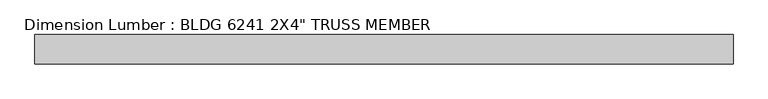
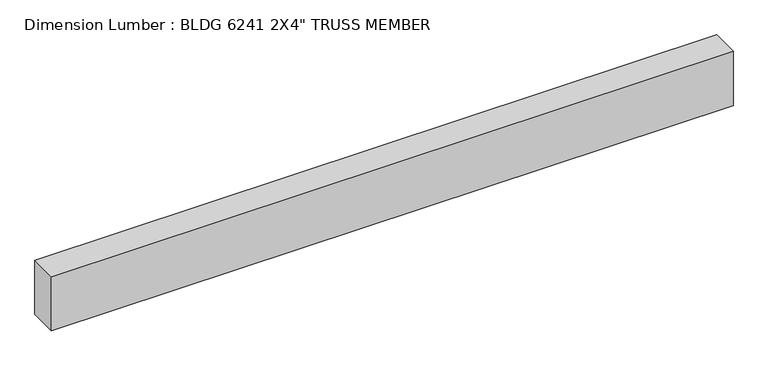
"""IFC4 building model written with IfcOpenShell, lengths in millimetres: beam geometry."""

from ifc_helpers import new_model, si_unit, frame, origin, place, context, project, spatial, polyline, outline, extrude, source, transform, mapped, element, save


def beam_85682148(model_context):
    return source(origin(), model_context, "Body", "SweptSolid", [
        extrude(outline(polyline([(595.8662636, -25.4), (-609.6, -25.4), (-609.6, 25.4), (595.8662636, 25.4), (595.8662636, -25.4)])), frame((0.0, 0.0, -50.8), z_axis=(0.0, 0.0, 1.0), x_axis=(1.0, 0.0, 0.0)), (0.0, 0.0, 1.0), 101.6),
    ])


if __name__ == "__main__":
    model = new_model("IFC4")
    model_context = context("Model", 3, world=origin())
    ifc_project = project(units=[si_unit("LENGTHUNIT", "METRE", prefix="MILLI")], contexts=[model_context])
    site = spatial("IfcSite", under=ifc_project)
    building = spatial("IfcBuilding", under=site)
    placement = place(None, origin())
    beam_shape = beam_85682148(model_context)
    element("IfcBeam", 1, ObjectType="Dimension Lumber : BLDG 6241 2X4\" TRUSS MEMBER", at=placement, inside=building, context=model_context, shape_type="MappedRepresentation", body=[
        mapped(beam_shape, transform((0.0, 0.0, 0.0), x_axis=(1.0, 0.0, 0.0), y_axis=(0.0, 1.0, 0.0), z_axis=(0.0, 0.0, 1.0))),
    ])
    save(model, "model.ifc")

# Revit data of these elements
# Type "Dimension Lumber : BLDG 6241 2X4\" TRUSS MEMBER"
#   Assembly Code = "B10"
#   A = 0.273472 SF
#   Length [instance default] = 5' - 0"
#   b = 0' - 2"
#   d = 0' - 4"
#   Structural Material [instance default] = Softwood, Lumber
# Element 1 (IfcBeam, "Dimension Lumber : BLDG 6241 2X4\" TRUSS MEMBER")
#   Materials on its faces: "Softwood, Lumber"
# Materials
#   "Softwood, Lumber": class "Wood", colour RGB 223 192 134, transparency 0, Description = "Pinus Echinata", Cost = 0
